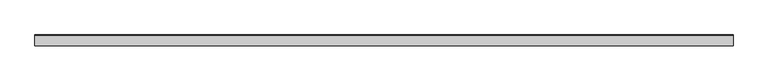
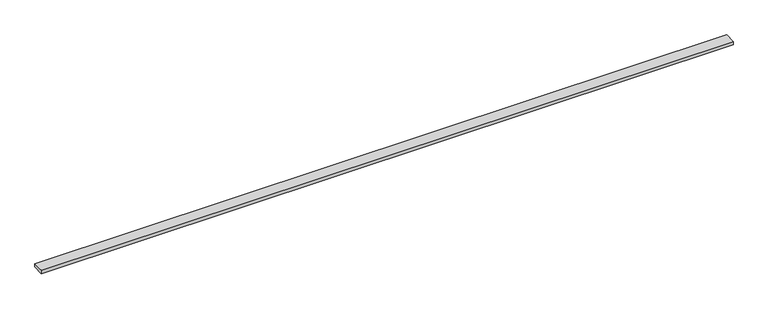
"""IFC4 building model written with IfcOpenShell, lengths in millimetres: proxy geometry, Inner panel:Inner panel:1:Inner panel:1 : Inner panel:Inner panel:300324:2:Inner panel:1:Inner panel:1 : Inner panel:Inner panel:300324:2 : Inner panel:Inner panel:1:Inner panel:1 : Inner panel:Inner panel:300324:300043:3 : Inner panel:Inner panel:1:Inner panel:1 : Inner panel:Inner panel:300324:2:Inner panel:1:Inner panel:1 : Inner panel:Inner panel:300324:2 : Inner panel:Inner panel:1:Inner panel:1 : Inner panel:Inner panel:300324:300043:308120."""

from ifc_helpers import new_model, si_unit, frame, origin, place, context, project, spatial, polyline, outline, extrude, source, transform, mapped, element, save


def generic_models_522a284c(model_context):
    return source(origin(), model_context, "Body", "SweptSolid", [
        extrude(outline(polyline([(0.0, -75.8934963), (0.0, 0.0), (4876.8, 0.0), (4876.8, -75.8934963), (0.0, -75.8934963)])), frame((596182.8367239, -575788.6771239, 4058.3102399), z_axis=(0.0, -0.04163054471215047, 0.9991330730923532), x_axis=(-1.0, 0.0, 0.0)), (0.0, 0.0, 1.0), 25.4),
    ])


if __name__ == "__main__":
    model = new_model("IFC4")
    model_context = context("Model", 3, world=origin())
    ifc_project = project(units=[si_unit("LENGTHUNIT", "METRE", prefix="MILLI")], contexts=[model_context])
    site = spatial("IfcSite", under=ifc_project)
    building = spatial("IfcBuilding", under=site)
    placement = place(None, origin())
    generic_models_shape = generic_models_522a284c(model_context)
    element("IfcBuildingElementProxy", 1, Name="Inner panel:Inner panel:1:Inner panel:1 : Inner panel:Inner panel:300324:2:Inner panel:1:Inner panel:1 : Inner panel:Inner panel:300324:2 : Inner panel:Inner panel:1:Inner panel:1 : Inner panel:Inner panel:300324:300043:3 : Inner panel:Inner panel:1:Inner panel:1 : Inner panel:Inner panel:300324:2:Inner panel:1:Inner panel:1 : Inner panel:Inner panel:300324:2 : Inner panel:Inner panel:1:Inner panel:1 : Inner panel:Inner panel:300324:300043:308120", ObjectType="Inner panel:Inner panel:1:Inner panel:1 : Inner panel:Inner panel:300324:2:Inner panel:1:Inner panel:1 : Inner panel:Inner panel:300324:2 : Inner panel:Inner panel:1:Inner panel:1 : Inner panel:Inner panel:300324:300043:3 : Inner panel:Inner panel:1:Inner panel:1 : Inner panel:Inner panel:300324:2:Inner panel:1:Inner panel:1 : Inner panel:Inner panel:300324:2 : Inner panel:Inner panel:1:Inner panel:1 : Inner panel:Inner panel:300324:300043:308120", at=placement, inside=building, context=model_context, shape_type="MappedRepresentation", body=[
        mapped(generic_models_shape, transform((0.0, 0.0, 0.0), x_axis=(1.0, 0.0, 0.0), y_axis=(0.0, 1.0, 0.0), z_axis=(0.0, 0.0, 1.0))),
    ])
    save(model, "model.ifc")

# Revit data of these elements
# Type "Inner panel:Inner panel:1:Inner panel:1 : Inner panel:Inner panel:300324:2:Inner panel:1:Inner panel:1 : Inner panel:Inner panel:300324:2 : Inner panel:Inner panel:1:Inner panel:1 : Inner panel:Inner panel:300324:300043:3 : Inner panel:Inner panel:1:Inner panel:1 : Inner panel:Inner panel:300324:2:Inner panel:1:Inner panel:1 : Inner panel:Inner panel:300324:2 : Inner panel:Inner panel:1:Inner panel:1 : Inner panel:Inner panel:300324:300043:308120"
#   NameOverride = "Inner panel:Inner panel:1:Inner panel:1 : Inner panel:Inner panel:300324:2:Inner panel:1:Inner panel:1 : Inner panel:Inner panel:300324:2 : Inner panel:Inner panel:1:Inner panel:1 : Inner panel:Inner panel:300324:300043:308120"
#   ObjectTypeOverride = "Inner panel:1:Inner panel:1 : Inner panel:Inner panel:300324:2 : Inner panel:Inner panel:1:Inner panel:1 : Inner panel:Inner panel:300324:300043"
#   Reference = "Inner panel"
#   Tag = "308120"
# Element 1 (IfcBuildingElementProxy, "Inner panel:Inner panel:1:Inner panel:1 : Inner panel:Inner panel:300324:2:Inner panel:1:Inner panel:1 : Inner panel:Inner panel:300324:2 : Inner panel:Inner panel:1:Inner panel:1 : Inner panel:Inner panel:300324:300043:3 : Inner panel:Inner panel:1:Inner panel:1 : Inner panel:Inner panel:300324:2:Inner panel:1:Inner panel:1 : Inner panel:Inner panel:300324:2 : Inner panel:Inner panel:1:Inner panel:1 : Inner panel:Inner panel:300324:300043:308120")
#   Materials on its faces: "1\" THERMAL SPACER @ PURLIN"
# Materials
#   "1\" THERMAL SPACER @ PURLIN": class "Unassigned", colour RGB 205 188 106, transparency 0, Cost = 0
